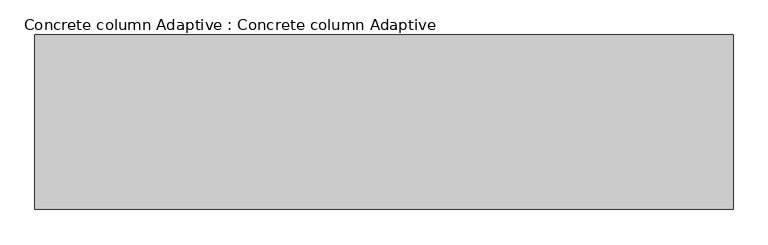
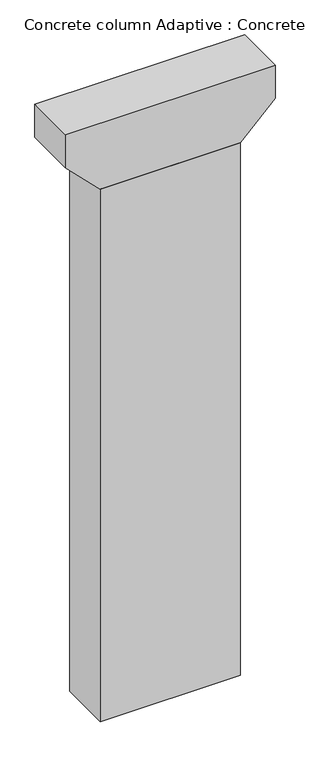
"""IFC4 building model written with IfcOpenShell, lengths in millimetres: proxy geometry, Concrete column Adaptive : Concrete column Adaptive."""

import ifcopenshell
import ifcopenshell.guid

model = None  # the IFC model being written
_history = None  # IfcOwnerHistory: only IFC2X3 demands one
_inside = {}  # id of a spatial element -> (the spatial element, [elements in it])
_under = {}  # id of a project, library or spatial element -> (it, [spatial elements below it])
_declared = {}  # id of a project -> (the project, [libraries it declares])
_typed = {}  # id of a type object -> (the type object, [elements of that type])
_made_of = {}  # id of a material, layer set ... -> (it, [elements and type objects made of it])


def new_model(schema):
    """Start an empty IFC model of exactly this schema.

    Asked for "IFC4X3", IfcOpenShell would pick the latest addendum, in which some entities
    have other attributes; the version numbers below select the first issue.
    IFC2X3 requires an IfcOwnerHistory on every rooted entity: one is made here for all.
    """
    global model, _history
    if schema == "IFC4X3":
        model = ifcopenshell.file(schema_version=(4, 3, 0, 0))
    else:
        model = ifcopenshell.file(schema=schema)
    _inside.clear()
    _under.clear()
    _declared.clear()
    _typed.clear()
    _made_of.clear()
    _history = None
    if model.schema == "IFC2X3":
        org = make("IfcOrganization", Name="unknown")
        user = make(
            "IfcPersonAndOrganization",
            ThePerson=make("IfcPerson", FamilyName="unknown"),
            TheOrganization=org,
        )
        app = make(
            "IfcApplication",
            ApplicationDeveloper=org,
            Version="unknown",
            ApplicationFullName="unknown",
            ApplicationIdentifier="unknown",
        )
        _history = make(
            "IfcOwnerHistory",
            OwningUser=user,
            OwningApplication=app,
            ChangeAction="ADDED",
            CreationDate=0,
        )
    return model


def make(cls, **values):
    """One entity of the class cls with the attributes given. An attribute that is None is left unset."""
    return model.create_entity(
        cls, **{name: value for name, value in values.items() if value is not None}
    )


def rooted(cls, **values):
    """An entity with a GlobalId (a new one), such as an element, a storey or a relation."""
    return make(cls, GlobalId=ifcopenshell.guid.new(), OwnerHistory=_history, **values)


def si_unit(unit_type, name, prefix=None):
    """IfcSIUnit, for example si_unit("LENGTHUNIT", "METRE", prefix="MILLI")."""
    return make("IfcSIUnit", UnitType=unit_type, Prefix=prefix, Name=name)


def assignment(units):
    """IfcUnitAssignment: the units of a project."""
    return None if units is None else make("IfcUnitAssignment", Units=units)


def point(xyz):
    """IfcCartesianPoint."""
    return None if xyz is None else make("IfcCartesianPoint", Coordinates=xyz)


def direction(xyz):
    """IfcDirection."""
    return None if xyz is None else make("IfcDirection", DirectionRatios=xyz)


def frame(location, z_axis=None, x_axis=None):
    """IfcAxis2Placement3D, a coordinate frame: its origin and axes. An axis left out is left unset."""
    return make(
        "IfcAxis2Placement3D",
        Location=point(location),
        Axis=direction(z_axis),
        RefDirection=direction(x_axis),
    )


def origin():
    """The frame at (0, 0, 0) with its axes left unset."""
    return frame((0.0, 0.0, 0.0))


def origin_with_axes():
    """The frame at (0, 0, 0) with the z axis (0, 0, 1) and the x axis (1, 0, 0) written out."""
    return frame((0.0, 0.0, 0.0), z_axis=(0.0, 0.0, 1.0), x_axis=(1.0, 0.0, 0.0))


def place(relative_to, where):
    """IfcLocalPlacement: puts the frame where relative to a parent placement (None: the world)."""
    return make(
        "IfcLocalPlacement", PlacementRelTo=relative_to, RelativePlacement=where
    )


def context(
    kind, dimensions, precision=None, world=None, true_north=None, identifier=None
):
    """IfcGeometricRepresentationContext, for example the 3D "Model" context."""
    return make(
        "IfcGeometricRepresentationContext",
        ContextIdentifier=identifier,
        ContextType=kind,
        CoordinateSpaceDimension=dimensions,
        Precision=precision,
        WorldCoordinateSystem=world,
        TrueNorth=true_north,
    )


def project(units=None, contexts=None):
    """IfcProject with its units and contexts."""
    return rooted(
        "IfcProject",
        Name="project",
        RepresentationContexts=contexts,
        UnitsInContext=assignment(units),
    )


def spatial(cls, under=None, at=None, **own):
    """A site, building, storey or space (cls), placed at a placement, below another one or the project."""
    s = rooted(cls, ObjectPlacement=at, **own)
    if under is not None:
        _under.setdefault(under.id(), (under, []))[1].append(s)
    return s


def polyline(points):
    """IfcPolyline through the points."""
    return make("IfcPolyline", Points=[point(p) for p in points])


def outline(outer, holes=None, kind="AREA"):
    """IfcArbitraryClosedProfileDef: a profile drawn as a closed curve; with holes, ...WithVoids."""
    if holes is None:
        return make("IfcArbitraryClosedProfileDef", ProfileType=kind, OuterCurve=outer)
    return make(
        "IfcArbitraryProfileDefWithVoids",
        ProfileType=kind,
        OuterCurve=outer,
        InnerCurves=holes,
    )


def extrude(swept, where, along, depth):
    """IfcExtrudedAreaSolid: the profile swept, set in the frame where, extruded along a direction by depth."""
    return make(
        "IfcExtrudedAreaSolid",
        SweptArea=swept,
        Position=where,
        ExtrudedDirection=direction(along),
        Depth=depth,
    )


def shape(context_of_items, identifier, shape_type, items):
    """IfcShapeRepresentation: the items that make up one representation, for example the "Body"."""
    return make(
        "IfcShapeRepresentation",
        ContextOfItems=context_of_items,
        RepresentationIdentifier=identifier,
        RepresentationType=shape_type,
        Items=items,
    )


def source(mapping_origin, context_of_items, identifier, shape_type, items):
    """IfcRepresentationMap: a shape defined once, which mapped items show again and again."""
    return make(
        "IfcRepresentationMap",
        MappingOrigin=mapping_origin,
        MappedRepresentation=shape(context_of_items, identifier, shape_type, items),
    )


def transform(
    local_origin,
    x_axis=None,
    y_axis=None,
    z_axis=None,
    scale=None,
    scale2=None,
    scale3=None,
    uniform=True,
):
    """IfcCartesianTransformationOperator3D, or its non-uniform kind. x_axis, y_axis, z_axis: its Axis1, 2, 3."""
    if uniform:
        return make(
            "IfcCartesianTransformationOperator3D",
            Axis1=direction(x_axis),
            Axis2=direction(y_axis),
            LocalOrigin=point(local_origin),
            Scale=scale,
            Axis3=direction(z_axis),
        )
    return make(
        "IfcCartesianTransformationOperator3DnonUniform",
        Axis1=direction(x_axis),
        Axis2=direction(y_axis),
        LocalOrigin=point(local_origin),
        Scale=scale,
        Axis3=direction(z_axis),
        Scale2=scale2,
        Scale3=scale3,
    )


def mapped(mapping_source, mapping_target):
    """IfcMappedItem: shows the shape of a source again, moved by a transform."""
    return make(
        "IfcMappedItem", MappingSource=mapping_source, MappingTarget=mapping_target
    )


def made_of(thing, what):
    """Note that an element or type object is made of a material, layer set ...; save() writes the relation."""
    if what is not None:
        _made_of.setdefault(what.id(), (what, []))[1].append(thing)
    return thing


def element(
    cls,
    number,
    at=None,
    inside=None,
    cuts=None,
    type_object=None,
    material=None,
    context=None,
    identifier="Body",
    shape_type=None,
    held_by="IfcProductDefinitionShape",
    body=None,
    shapes=None,
    **own,
):
    """One element of the class cls, such as IfcWall. Its Tag is "e" and its number.

    at: its placement. inside: the storey or other place that contains it. cuts: it is an
    opening in that element (IfcRelVoidsElement). A single representation is given by context,
    identifier, shape_type and body (its items); several are given by shapes. held_by: the class
    of the entity that holds the representations. save() writes the other relations.
    """
    e = rooted(cls, Tag="e%d" % number, ObjectPlacement=at, **own)
    if body is not None:
        shapes = [shape(context, identifier, shape_type, body)]
    if shapes is not None:
        e.Representation = make(held_by, Representations=shapes)
    if inside is not None:
        _inside.setdefault(inside.id(), (inside, []))[1].append(e)
    if cuts is not None:
        rooted(
            "IfcRelVoidsElement", RelatingBuildingElement=cuts, RelatedOpeningElement=e
        )
    if type_object is not None:
        _typed.setdefault(type_object.id(), (type_object, []))[1].append(e)
    return made_of(e, material)


def aggregate(whole, parts):
    """IfcRelAggregates: a whole, such as a stair, and the parts it consists of."""
    return rooted("IfcRelAggregates", RelatingObject=whole, RelatedObjects=parts)


def save(model, path):
    """Write the relations noted so far, then the file.

    IfcRelAggregates (storeys below a building ...), IfcRelContainedInSpatialStructure (elements
    in a storey), IfcRelDefinesByType, IfcRelAssociatesMaterial and IfcRelDeclares: one each for
    every whole, place, type object, material and project.
    """
    for whole, parts in _under.values():
        aggregate(whole, parts)
    for where, things in _inside.values():
        rooted(
            "IfcRelContainedInSpatialStructure",
            RelatedElements=things,
            RelatingStructure=where,
        )
    for kind, things in _typed.values():
        rooted("IfcRelDefinesByType", RelatedObjects=things, RelatingType=kind)
    for what, things in _made_of.values():
        rooted("IfcRelAssociatesMaterial", RelatedObjects=things, RelatingMaterial=what)
    for by, libraries in _declared.values():
        rooted("IfcRelDeclares", RelatingContext=by, RelatedDefinitions=libraries)
    model.write(path)


def concrete_column_adaptive_concrete_column_adaptive_8623096c(model_context):
    return source(origin(), model_context, "Body", "SweptSolid", [
        extrude(outline(polyline([(36183.0, 6000.0), (36183.0, -6000.0), (34183.0, -6000.0), (32183.0, -4000.0), (32183.0, 4000.0), (34183.0, 6000.0), (36183.0, 6000.0)])), frame((0.0, -1500.0, 0.0), z_axis=(0.0, 1.0, 0.0), x_axis=(0.0, 0.0, 1.0)), (0.0, 0.0, 1.0), 3000.0),
        extrude(outline(polyline([(-4000.0, -1500.0), (-4000.0, 1500.0), (4000.0, 1500.0), (4000.0, -1500.0), (-4000.0, -1500.0)])), origin_with_axes(), (0.0, 0.0, 1.0), 32183.0),
    ])


if __name__ == "__main__":
    model = new_model("IFC4")
    model_context = context("Model", 3, world=origin())
    ifc_project = project(units=[si_unit("LENGTHUNIT", "METRE", prefix="MILLI")], contexts=[model_context])
    site = spatial("IfcSite", under=ifc_project)
    building = spatial("IfcBuilding", under=site)
    placement = place(None, origin())
    concrete_column_adaptive_concrete_column_adaptive_shape = concrete_column_adaptive_concrete_column_adaptive_8623096c(model_context)
    element("IfcBuildingElementProxy", 1, Name="Concrete column Adaptive : Concrete column Adaptive", ObjectType="Concrete column Adaptive : Concrete column Adaptive", at=placement, inside=building, context=model_context, shape_type="MappedRepresentation", body=[
        mapped(concrete_column_adaptive_concrete_column_adaptive_shape, transform((0.0, 0.0, 0.0), x_axis=(1.0, 0.0, 0.0), y_axis=(0.0, 1.0, 0.0), z_axis=(0.0, 0.0, 1.0))),
    ])
    save(model, "model.ifc")

# Revit data of these elements
# Type "Concrete column Adaptive : Concrete column Adaptive"
#   Height [instance default] = 30000 mm
#   Default Elevation = 0
# Element 1 (IfcBuildingElementProxy, "Concrete column Adaptive : Concrete column Adaptive")
#   Height = 32183 mm
